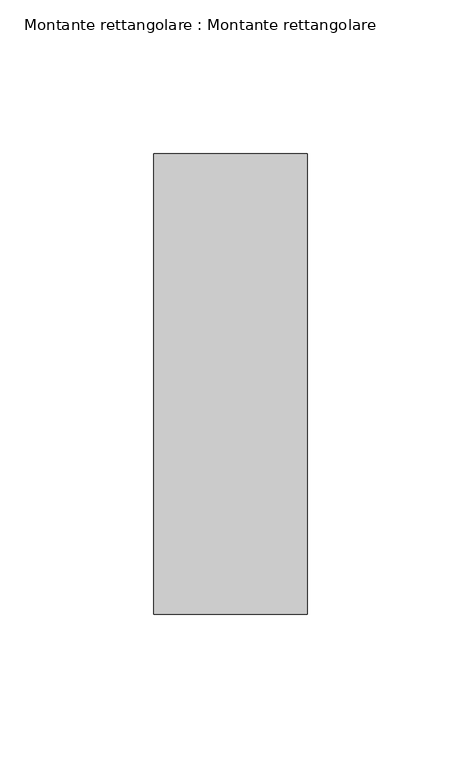
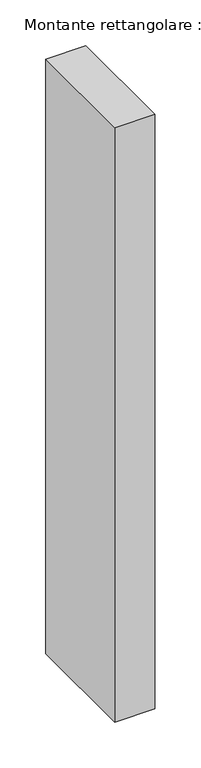
"""IFC4 building model written with IfcOpenShell, lengths in millimetres: member geometry, Montante rettangolare : Montante rettangolare."""

from ifc_helpers import new_model, si_unit, frame, origin, place, context, project, spatial, polyline, outline, extrude, source, transform, mapped, element, save


def montante_rettangolare_montante_rettangolare_81407c8a(model_context):
    return source(origin(), model_context, "Body", "SweptSolid", [
        extrude(outline(polyline([(0.0, 75.0), (0.0, -75.0), (-50.0, -75.0), (-50.0, 75.0), (0.0, 75.0)])), frame((0.0, 0.0, -790.0), z_axis=(0.0, 0.0, 1.0), x_axis=(1.0, 0.0, 0.0)), (0.0, 0.0, 1.0), 790.0),
    ])


if __name__ == "__main__":
    model = new_model("IFC4")
    model_context = context("Model", 3, world=origin())
    ifc_project = project(units=[si_unit("LENGTHUNIT", "METRE", prefix="MILLI")], contexts=[model_context])
    site = spatial("IfcSite", under=ifc_project)
    building = spatial("IfcBuilding", under=site)
    placement = place(None, origin())
    montante_rettangolare_montante_rettangolare_shape = montante_rettangolare_montante_rettangolare_81407c8a(model_context)
    element("IfcMember", 1, ObjectType="Montante rettangolare : Montante rettangolare", at=placement, inside=building, context=model_context, shape_type="MappedRepresentation", body=[
        mapped(montante_rettangolare_montante_rettangolare_shape, transform((0.0, 0.0, 0.0), x_axis=(1.0, 0.0, 0.0), y_axis=(0.0, 1.0, 0.0), z_axis=(0.0, 0.0, 1.0))),
    ])
    save(model, "model.ifc")

# Revit data of these elements
# Type "Montante rettangolare : Montante rettangolare"
#   built-in parameter 1007304 = 0.492126 (stored number, unit not read)
#   built-in parameter 1007301 = 0.082021 (stored number, unit not read)
#   built-in parameter 1007300 = 0.082021 (stored number, unit not read)
# Element 1 (IfcMember, "Montante rettangolare : Montante rettangolare")
#   Materials on its faces: "Acciaio"
# Materials
#   "Acciaio": class "Metallo", colour RGB 247 247 247, transparency 0, Description = "Acciaio, finitura zigrinata", Cost = 0
